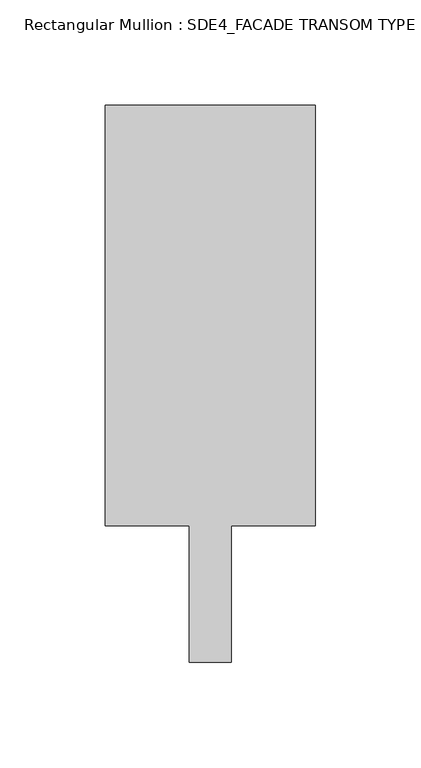
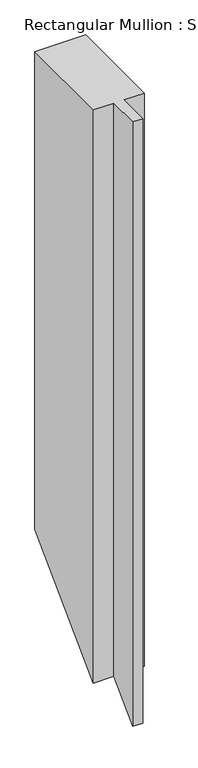
"""IFC4 building model written with IfcOpenShell, lengths in millimetres: member geometry, Rectangular Mullion : SDE4_FACADE TRANSOM TYPE 2."""

from ifc_helpers import new_model, si_unit, origin, place, context, project, spatial, faceted_brep, source, transform, mapped, element, save


def rectangular_mullion_sde4_facade_transom_type_2_fed565b7(model_context):
    return source(origin(), model_context, "Body", "Brep", [
        faceted_brep([(50.0, 132.5, 0.0), (-50.0, 132.5, 0.0), (-50.0, -67.5, 0.0), (-10.0, -67.5, 0.0), (-10.0, -132.5, 0.0), (10.0, -132.5, 0.0), (10.0, -67.5, 0.0), (50.0, -67.5, 0.0), (50.0, 132.5, -996.875), (-50.0, 132.5, -996.875), (-50.0, -67.5, -1196.875), (-10.0, -67.5, -1196.875), (-10.0, -132.5, -1261.875), (10.0, -132.5, -1261.875), (10.0, -67.5, -1196.875), (50.0, -67.5, -1196.875)], [[[0, 1, 2, 3, 4, 5, 6, 7]], [[1, 0, 8, 9]], [[2, 1, 9, 10]], [[3, 2, 10, 11]], [[4, 3, 11, 12]], [[5, 4, 12, 13]], [[6, 5, 13, 14]], [[7, 6, 14, 15]], [[0, 7, 15, 8]], [[8, 15, 14, 13, 12, 11, 10, 9]]]),
    ])


if __name__ == "__main__":
    model = new_model("IFC4")
    model_context = context("Model", 3, world=origin())
    ifc_project = project(units=[si_unit("LENGTHUNIT", "METRE", prefix="MILLI")], contexts=[model_context])
    site = spatial("IfcSite", under=ifc_project)
    building = spatial("IfcBuilding", under=site)
    placement = place(None, origin())
    rectangular_mullion_sde4_facade_transom_type_2_shape = rectangular_mullion_sde4_facade_transom_type_2_fed565b7(model_context)
    element("IfcMember", 1, ObjectType="Rectangular Mullion : SDE4_FACADE TRANSOM TYPE 2", at=placement, inside=building, context=model_context, shape_type="MappedRepresentation", body=[
        mapped(rectangular_mullion_sde4_facade_transom_type_2_shape, transform((0.0, 0.0, 0.0), x_axis=(1.0, 0.0, 0.0), y_axis=(0.0, 1.0, 0.0), z_axis=(0.0, 0.0, 1.0))),
    ])
    save(model, "model.ifc")

# Revit data of these elements
# Type "Rectangular Mullion : SDE4_FACADE TRANSOM TYPE 2"
#   built-in parameter 1007322 = 0.869423 (stored number, unit not read)
#   built-in parameter 1007321 = 0.164042 (stored number, unit not read)
#   built-in parameter 1007320 = 0.164042 (stored number, unit not read)
